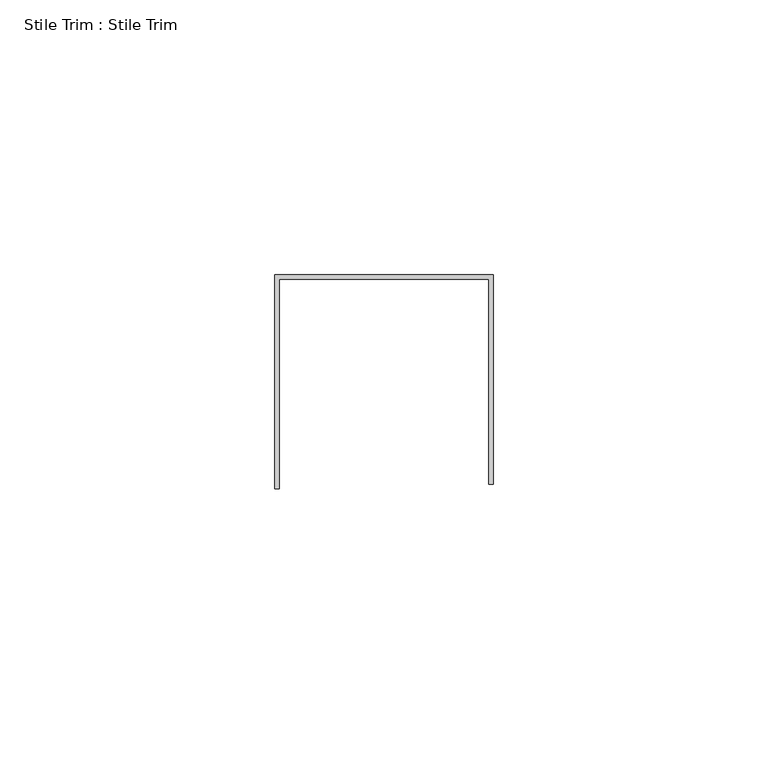
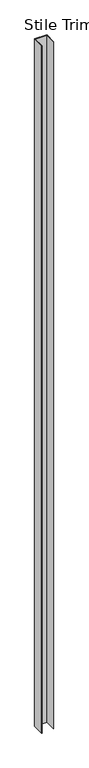
"""IFC4 building model written with IfcOpenShell, lengths in millimetres: proxy geometry, Stile Trim : Stile Trim."""

from ifc_helpers import new_model, si_unit, frame, origin, place, context, project, spatial, polyline, outline, extrude, source, transform, mapped, element, save


def stile_trim_stile_trim_02668cd7(model_context):
    return source(origin(), model_context, "Body", "SweptSolid", [
        extrude(outline(polyline([(587327.0060739, -531784.4789841), (587366.6808739, -531784.4789841), (587366.6808739, -531822.5789841), (587365.8934739, -531822.5789841), (587365.8934739, -531785.2663841), (587327.7934739, -531785.2663841), (587327.7934739, -531823.3663841), (587327.0060739, -531823.3663841), (587327.0060739, -531784.4789841)])), frame((0.0, 0.0, 50.8), z_axis=(0.0, 0.0, 1.0), x_axis=(1.0, 0.0, 0.0)), (0.0, 0.0, 1.0), 2350.3929688),
    ])


if __name__ == "__main__":
    model = new_model("IFC4")
    model_context = context("Model", 3, world=origin())
    ifc_project = project(units=[si_unit("LENGTHUNIT", "METRE", prefix="MILLI")], contexts=[model_context])
    site = spatial("IfcSite", under=ifc_project)
    building = spatial("IfcBuilding", under=site)
    placement = place(None, origin())
    stile_trim_stile_trim_shape = stile_trim_stile_trim_02668cd7(model_context)
    element("IfcBuildingElementProxy", 1, Name="Stile Trim : Stile Trim", ObjectType="Stile Trim : Stile Trim", at=placement, inside=building, context=model_context, shape_type="MappedRepresentation", body=[
        mapped(stile_trim_stile_trim_shape, transform((0.0, 0.0, 0.0), x_axis=(1.0, 0.0, 0.0), y_axis=(0.0, 1.0, 0.0), z_axis=(0.0, 0.0, 1.0))),
    ])
    save(model, "model.ifc")

# Revit data of these elements
# Element 1 (IfcBuildingElementProxy, "Stile Trim : Stile Trim")
#   Materials on its faces: "EDGE TRIM BY MTL PANEL MFR."
# Materials
#   "EDGE TRIM BY MTL PANEL MFR.": class "Generic", colour RGB 239 242 240, transparency 0, Cost = 0
